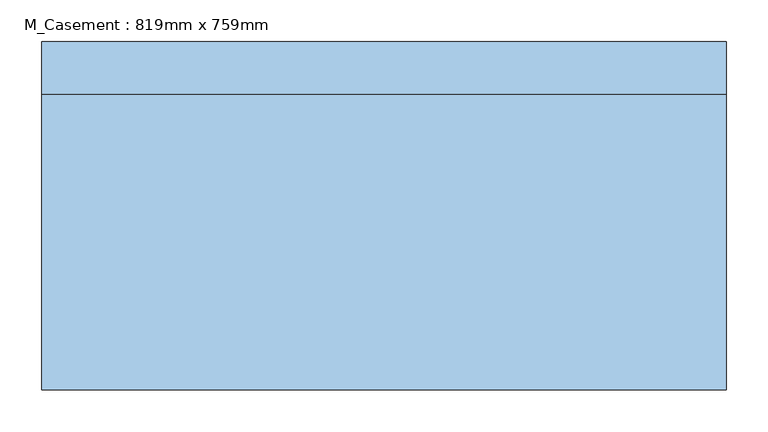
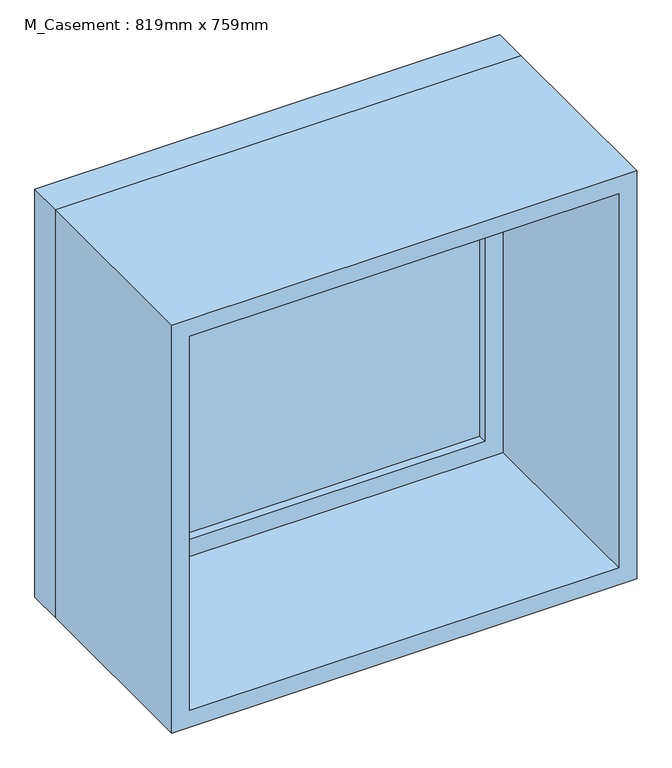
"""IFC4 building model written with IfcOpenShell, lengths in millimetres: window geometry, M_Casement : 819mm x 759mm."""

from ifc_helpers import new_model, si_unit, frame, origin, place, context, project, spatial, polyline, outline, extrude, source, transform, mapped, element, save


def m_casement_819mm_x_759mm_6ad0bdaf(model_context):
    return source(origin(), model_context, "Body", "SweptSolid", [
        extrude(outline(polyline([(346.0, 160.925), (-346.0, 160.925), (-346.0, 173.625), (346.0, 173.625), (346.0, 160.925)])), frame((0.0, 0.0, 978.5), z_axis=(0.0, 0.0, 1.0), x_axis=(1.0, 0.0, 0.0)), (0.0, 0.0, 1.0), 632.0),
        extrude(outline(polyline([(1654.95, -390.45), (934.05, -390.45), (934.05, 390.45), (1654.95, 390.45), (1654.95, -390.45)]), holes=[polyline([(1610.5, -346.0), (1610.5, 346.0), (978.5, 346.0), (978.5, -346.0), (1610.5, -346.0)])]), frame((0.0, 145.05, 0.0), z_axis=(0.0, 1.0, 0.0), x_axis=(0.0, 0.0, 1.0)), (0.0, 0.0, 1.0), 44.45),
        extrude(outline(polyline([(1674.0, -409.5), (915.0, -409.5), (915.0, 409.5), (1674.0, 409.5), (1674.0, -409.5)]), holes=[polyline([(1642.25, -377.75), (1642.25, 377.75), (946.75, 377.75), (946.75, -377.75), (1642.25, -377.75)])]), frame((0.0, -208.5, 0.0), z_axis=(0.0, 1.0, 0.0), x_axis=(0.0, 0.0, 1.0)), (0.0, 0.0, 1.0), 353.55),
        extrude(outline(polyline([(1674.0, 409.5), (1674.0, -409.5), (915.0, -409.5), (915.0, 409.5), (1674.0, 409.5)]), holes=[polyline([(1654.95, 390.45), (934.05, 390.45), (934.05, -390.45), (1654.95, -390.45), (1654.95, 390.45)])]), frame((0.0, 145.05, 0.0), z_axis=(0.0, 1.0, 0.0), x_axis=(0.0, 0.0, 1.0)), (0.0, 0.0, 1.0), 63.45),
    ])


if __name__ == "__main__":
    model = new_model("IFC4")
    model_context = context("Model", 3, world=origin())
    ifc_project = project(units=[si_unit("LENGTHUNIT", "METRE", prefix="MILLI")], contexts=[model_context])
    site = spatial("IfcSite", under=ifc_project)
    building = spatial("IfcBuilding", under=site)
    placement = place(None, origin())
    m_casement_819mm_x_759mm_shape = m_casement_819mm_x_759mm_6ad0bdaf(model_context)
    element("IfcWindow", 1, ObjectType="M_Casement : 819mm x 759mm", at=placement, inside=building, context=model_context, shape_type="MappedRepresentation", body=[
        mapped(m_casement_819mm_x_759mm_shape, transform((0.0, 0.0, 0.0), x_axis=(1.0, 0.0, 0.0), y_axis=(0.0, 1.0, 0.0), z_axis=(0.0, 0.0, 1.0))),
    ])
    save(model, "model.ifc")

# Revit data of these elements
# Type "M_Casement : 819mm x 759mm"
#   Manufacturer = "Manufacturer"
#   Type Mark = "03"
#   Construction Type = "Construction Type"
#   AccessibilityPerformance = "AccessibilityPerformance"
#   CodePerformance = "CodePerformance"
#   ConfigurationType = "ConfigurationType"
#   ConstructionType = "ConstructionType"
#   FireRating = "FireRating"
#   GlazingAreaFraction = "GlazingAreaFraction"
#   OperationType = "OperationType"
#   Area = "Area"
#   Color = "Color"
#   Constituents = "Constituents"
#   Features = "Features"
#   Finish = "Finish"
#   Grade = "Grade"
#   Material = "Material"
#   ModelReference = "ModelReference"
#   NominalHeight = "NominalHeight"
#   NominalLength = "NominalLength"
#   NominalWidth = "NominalWidth"
#   ProductionYear = "ProductionYear"
#   Reference = "Reference"
#   Shape = "Shape"
#   Size = "Size"
#   SustainabilityPerformance = "SustainabilityPerformance"
#   WarrantyDescription = "WarrantyDescription"
#   WarrantyDurationLabor = "WarrantyDurationLabor"
#   WarrantyDurationParts = "WarrantyDurationParts"
#   WarrantyGuarantorLabor = "WarrantyGuarantorLabor"
#   WarrantyGuarantorParts = "WarrantyGuarantorParts"
#   ExpectedLife = "ExpectedLife"
#   ReplacementCost = "ReplacementCost"
#   AssetAccountingType = "FIXED"
#   ModelLabel = "ModelLabel"
#   Height = 0.759 m
#   Default Sill Height = 0.915 m
#   Width = 0.819 m
#   Window Inset = 0.019 m
#   Glass Pane Material = Glass
#   Sash = Sash
#   Trim Exterior Material = Trim
#   Trim Interior Material = Trim
#   Wall Closure = (empty or 0)
# Element 1 (IfcWindow, "M_Casement : 819mm x 759mm")
#   Materials on its faces: "Trim", "Sash", "Glass"
# Materials
#   "Glass": class "Glass", colour RGB 0 128 192, transparency 0.9
#   "Sash": class "Wood", colour RGB 224 178 126, transparency 0
#   "Trim": class "Wood", colour RGB 224 178 126, transparency 0
